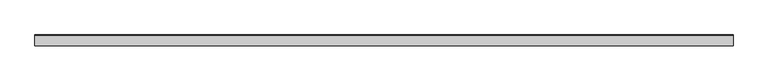
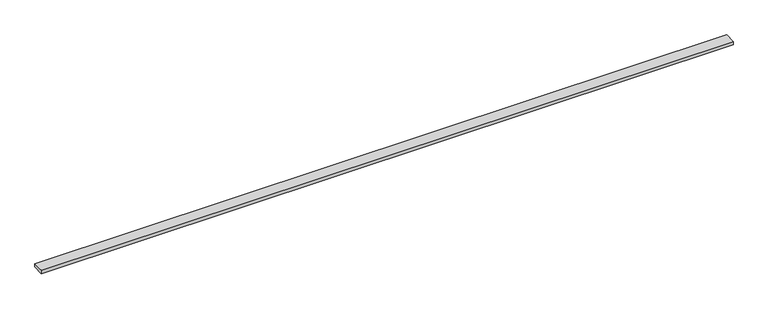
"""IFC4 building model written with IfcOpenShell, lengths in millimetres: proxy geometry, Inner panel:Inner panel:1:Inner panel:1 : Inner panel:Inner panel:300324:2:Inner panel:1:Inner panel:1 : Inner panel:Inner panel:300324:2 : Inner panel:Inner panel:1:Inner panel:1 : Inner panel:Inner panel:300324:300043:17 : Inner panel:Inner panel:1:Inner panel:1 : Inner panel:Inner panel:300324:2:Inner panel:1:Inner panel:1 : Inner panel:Inner panel:300324:2 : Inner panel:Inner panel:1:Inner panel:1 : Inner panel:Inner panel:300324:300043:308120."""

from ifc_helpers import new_model, si_unit, frame, origin, place, context, project, spatial, polyline, outline, extrude, source, transform, mapped, element, save


def generic_models_eaeba437(model_context):
    return source(origin(), model_context, "Body", "SweptSolid", [
        extrude(outline(polyline([(0.0, -75.8934963), (0.0, 0.0), (4876.8, 0.0), (4876.8, -75.8934963), (0.0, -75.8934963)])), frame((596182.8367242, -563785.2339734, 8961.6658909), z_axis=(0.0, -0.04163054471214335, 0.9991330730923536), x_axis=(-1.0, 0.0, 0.0)), (0.0, 0.0, 1.0), 25.4),
    ])


if __name__ == "__main__":
    model = new_model("IFC4")
    model_context = context("Model", 3, world=origin())
    ifc_project = project(units=[si_unit("LENGTHUNIT", "METRE", prefix="MILLI")], contexts=[model_context])
    site = spatial("IfcSite", under=ifc_project)
    building = spatial("IfcBuilding", under=site)
    placement = place(None, origin())
    generic_models_shape = generic_models_eaeba437(model_context)
    element("IfcBuildingElementProxy", 1, Name="Inner panel:Inner panel:1:Inner panel:1 : Inner panel:Inner panel:300324:2:Inner panel:1:Inner panel:1 : Inner panel:Inner panel:300324:2 : Inner panel:Inner panel:1:Inner panel:1 : Inner panel:Inner panel:300324:300043:17 : Inner panel:Inner panel:1:Inner panel:1 : Inner panel:Inner panel:300324:2:Inner panel:1:Inner panel:1 : Inner panel:Inner panel:300324:2 : Inner panel:Inner panel:1:Inner panel:1 : Inner panel:Inner panel:300324:300043:308120", ObjectType="Inner panel:Inner panel:1:Inner panel:1 : Inner panel:Inner panel:300324:2:Inner panel:1:Inner panel:1 : Inner panel:Inner panel:300324:2 : Inner panel:Inner panel:1:Inner panel:1 : Inner panel:Inner panel:300324:300043:17 : Inner panel:Inner panel:1:Inner panel:1 : Inner panel:Inner panel:300324:2:Inner panel:1:Inner panel:1 : Inner panel:Inner panel:300324:2 : Inner panel:Inner panel:1:Inner panel:1 : Inner panel:Inner panel:300324:300043:308120", at=placement, inside=building, context=model_context, shape_type="MappedRepresentation", body=[
        mapped(generic_models_shape, transform((0.0, 0.0, 0.0), x_axis=(1.0, 0.0, 0.0), y_axis=(0.0, 1.0, 0.0), z_axis=(0.0, 0.0, 1.0))),
    ])
    save(model, "model.ifc")

# Revit data of these elements
# Type "Inner panel:Inner panel:1:Inner panel:1 : Inner panel:Inner panel:300324:2:Inner panel:1:Inner panel:1 : Inner panel:Inner panel:300324:2 : Inner panel:Inner panel:1:Inner panel:1 : Inner panel:Inner panel:300324:300043:17 : Inner panel:Inner panel:1:Inner panel:1 : Inner panel:Inner panel:300324:2:Inner panel:1:Inner panel:1 : Inner panel:Inner panel:300324:2 : Inner panel:Inner panel:1:Inner panel:1 : Inner panel:Inner panel:300324:300043:308120"
#   NameOverride = "Inner panel:Inner panel:1:Inner panel:1 : Inner panel:Inner panel:300324:2:Inner panel:1:Inner panel:1 : Inner panel:Inner panel:300324:2 : Inner panel:Inner panel:1:Inner panel:1 : Inner panel:Inner panel:300324:300043:308120"
#   ObjectTypeOverride = "Inner panel:1:Inner panel:1 : Inner panel:Inner panel:300324:2 : Inner panel:Inner panel:1:Inner panel:1 : Inner panel:Inner panel:300324:300043"
#   Reference = "Inner panel"
#   Tag = "308120"
# Element 1 (IfcBuildingElementProxy, "Inner panel:Inner panel:1:Inner panel:1 : Inner panel:Inner panel:300324:2:Inner panel:1:Inner panel:1 : Inner panel:Inner panel:300324:2 : Inner panel:Inner panel:1:Inner panel:1 : Inner panel:Inner panel:300324:300043:17 : Inner panel:Inner panel:1:Inner panel:1 : Inner panel:Inner panel:300324:2:Inner panel:1:Inner panel:1 : Inner panel:Inner panel:300324:2 : Inner panel:Inner panel:1:Inner panel:1 : Inner panel:Inner panel:300324:300043:308120")
#   Materials on its faces: "1\" THERMAL SPACER @ PURLIN"
# Materials
#   "1\" THERMAL SPACER @ PURLIN": class "Unassigned", colour RGB 205 188 106, transparency 0, Cost = 0
